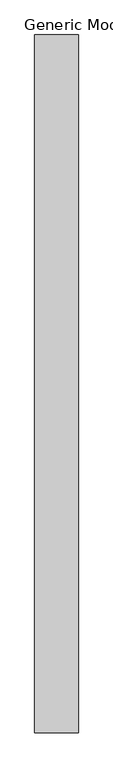
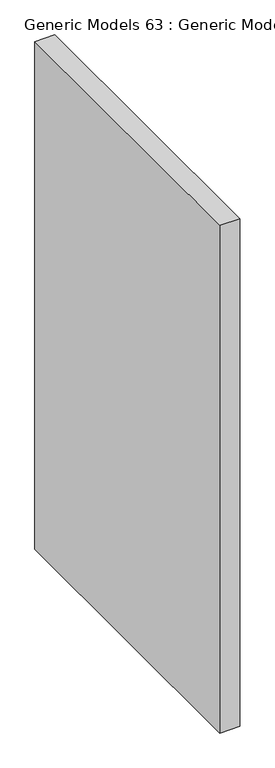
"""IFC4 building model written with IfcOpenShell, lengths in millimetres: proxy geometry, Generic Models 63 : Generic Models 1."""

from ifc_helpers import new_model, si_unit, frame, origin, place, context, project, spatial, polyline, outline, extrude, source, transform, mapped, element, save


def generic_models_63_generic_models_1_f1177d32(model_context):
    return source(origin(), model_context, "Body", "SweptSolid", [
        extrude(outline(polyline([(50996.85, 1219.2), (50996.85, 0.0), (50920.65, 0.0), (50920.65, 1219.2), (50996.85, 1219.2)])), frame((0.0, 0.0, 3090.8625), z_axis=(0.0, 0.0, 1.0), x_axis=(1.0, 0.0, 0.0)), (0.0, 0.0, 1.0), 2044.7),
    ])


if __name__ == "__main__":
    model = new_model("IFC4")
    model_context = context("Model", 3, world=origin())
    ifc_project = project(units=[si_unit("LENGTHUNIT", "METRE", prefix="MILLI")], contexts=[model_context])
    site = spatial("IfcSite", under=ifc_project)
    building = spatial("IfcBuilding", under=site)
    placement = place(None, origin())
    generic_models_63_generic_models_1_shape = generic_models_63_generic_models_1_f1177d32(model_context)
    element("IfcBuildingElementProxy", 1, Name="Generic Models 63 : Generic Models 1", ObjectType="Generic Models 63 : Generic Models 1", at=placement, inside=building, context=model_context, shape_type="MappedRepresentation", body=[
        mapped(generic_models_63_generic_models_1_shape, transform((0.0, 0.0, 0.0), x_axis=(1.0, 0.0, 0.0), y_axis=(0.0, 1.0, 0.0), z_axis=(0.0, 0.0, 1.0))),
    ])
    save(model, "model.ifc")

# Revit data of these elements
# Element 1 (IfcBuildingElementProxy, "Generic Models 63 : Generic Models 1")
#   Materials on its faces: "(S) SOUND BATT. INSULATION (THICKNESS TO MATCH WALL DEPTH)"
# Materials
#   "(S) SOUND BATT. INSULATION (THICKNESS TO MATCH WALL DEPTH)": class "Unassigned", colour RGB 255 255 255, transparency 0, Cost = 0
